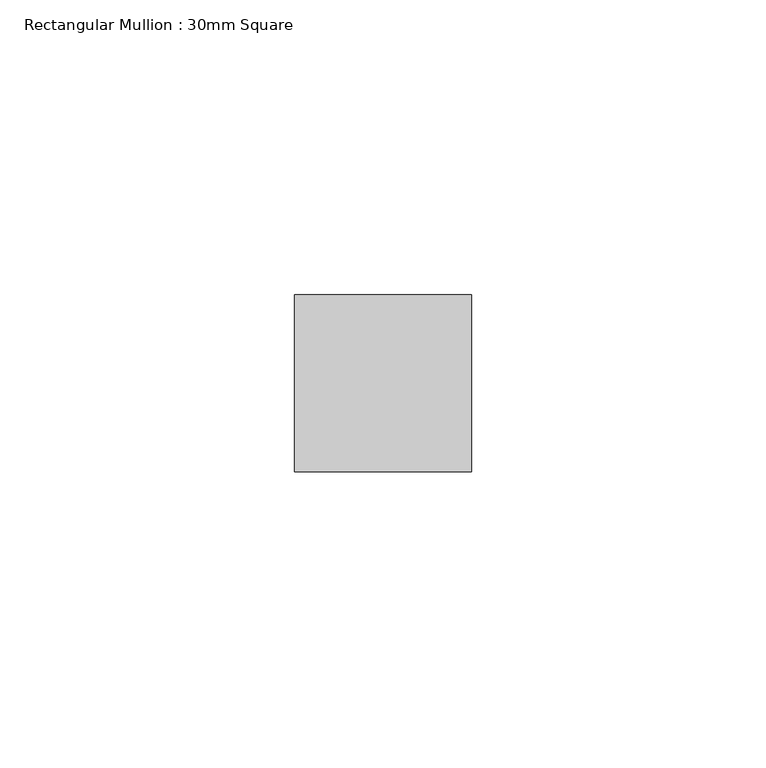
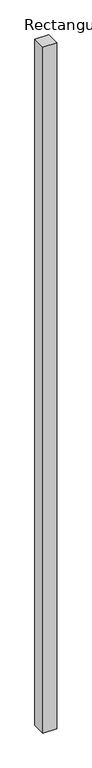
"""IFC4 building model written with IfcOpenShell, lengths in millimetres: member geometry, Rectangular Mullion : 30mm Square."""

from ifc_helpers import new_model, si_unit, frame, origin, place, context, project, spatial, polyline, outline, extrude, source, transform, mapped, element, save


def rectangular_mullion_30mm_square_9adde6a4(model_context):
    return source(origin(), model_context, "Body", "SweptSolid", [
        extrude(outline(polyline([(15.0, 15.0), (15.0, -15.0), (-15.0, -15.0), (-15.0, 15.0), (15.0, 15.0)])), frame((0.0, 0.0, -1575.8133586), z_axis=(0.0, 0.0, 1.0), x_axis=(1.0, 0.0, 0.0)), (0.0, 0.0, 1.0), 1575.8133586),
    ])


if __name__ == "__main__":
    model = new_model("IFC4")
    model_context = context("Model", 3, world=origin())
    ifc_project = project(units=[si_unit("LENGTHUNIT", "METRE", prefix="MILLI")], contexts=[model_context])
    site = spatial("IfcSite", under=ifc_project)
    building = spatial("IfcBuilding", under=site)
    placement = place(None, origin())
    rectangular_mullion_30mm_square_shape = rectangular_mullion_30mm_square_9adde6a4(model_context)
    element("IfcMember", 1, ObjectType="Rectangular Mullion : 30mm Square", at=placement, inside=building, context=model_context, shape_type="MappedRepresentation", body=[
        mapped(rectangular_mullion_30mm_square_shape, transform((0.0, 0.0, 0.0), x_axis=(1.0, 0.0, 0.0), y_axis=(0.0, 1.0, 0.0), z_axis=(0.0, 0.0, 1.0))),
    ])
    save(model, "model.ifc")

# Revit data of these elements
# Type "Rectangular Mullion : 30mm Square"
#   built-in parameter 1007304 = 0.0984252 (stored number, unit not read)
#   built-in parameter 1007301 = 0.0492126 (stored number, unit not read)
#   built-in parameter 1007300 = 0.0492126 (stored number, unit not read)
# Element 1 (IfcMember, "Rectangular Mullion : 30mm Square")
#   Materials on its faces: "Aluminum"
# Materials
#   "Aluminum": class "Metal", colour RGB 244 244 244, transparency 0, Description = "Aluminum 6061", Cost = 0
